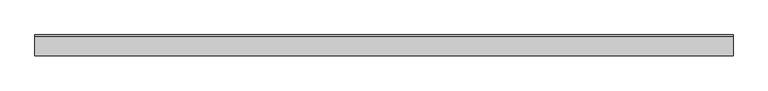
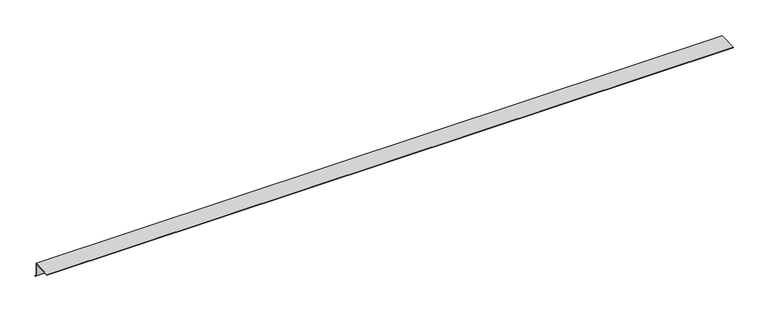
"""IFC4 building model written with IfcOpenShell, lengths in millimetres: proxy geometry, Generic Models 7:Generic Models 1:337419:Generic Models 1:337419 : Generic Models 7:Generic Models 1:337419:24 : Generic Models 7:Generic Models 1:337419:Generic Models 1:337419 : Generic Models 7:Generic Models 1:337419:301336."""

from ifc_helpers import new_model, si_unit, frame, origin, place, context, project, spatial, polyline, outline, extrude, source, transform, mapped, element, save


def generic_models_96069dc9(model_context):
    return source(origin(), model_context, "Body", "SweptSolid", [
        extrude(outline(polyline([(-536591.4802062, 10176.5740713), (-536591.5958611, 10179.3497879), (-536459.9713089, 10184.8341442), (-536459.9713089, 10095.8159785), (-536446.5009248, 10082.3455943), (-536448.4653558, 10080.3811633), (-536462.7494339, 10094.6652414), (-536462.7494339, 10181.9378535), (-536591.4802062, 10176.5740713)])), frame((591306.0367242, 0.0, 0.0), z_axis=(1.0, 0.0, 0.0), x_axis=(0.0, 1.0, 0.0)), (0.0, 0.0, 1.0), 4876.8),
    ])


if __name__ == "__main__":
    model = new_model("IFC4")
    model_context = context("Model", 3, world=origin())
    ifc_project = project(units=[si_unit("LENGTHUNIT", "METRE", prefix="MILLI")], contexts=[model_context])
    site = spatial("IfcSite", under=ifc_project)
    building = spatial("IfcBuilding", under=site)
    placement = place(None, origin())
    generic_models_shape = generic_models_96069dc9(model_context)
    element("IfcBuildingElementProxy", 1, Name="Generic Models 7:Generic Models 1:337419:Generic Models 1:337419 : Generic Models 7:Generic Models 1:337419:24 : Generic Models 7:Generic Models 1:337419:Generic Models 1:337419 : Generic Models 7:Generic Models 1:337419:301336", ObjectType="Generic Models 7:Generic Models 1:337419:Generic Models 1:337419 : Generic Models 7:Generic Models 1:337419:24 : Generic Models 7:Generic Models 1:337419:Generic Models 1:337419 : Generic Models 7:Generic Models 1:337419:301336", at=placement, inside=building, context=model_context, shape_type="MappedRepresentation", body=[
        mapped(generic_models_shape, transform((0.0, 0.0, 0.0), x_axis=(1.0, 0.0, 0.0), y_axis=(0.0, 1.0, 0.0), z_axis=(0.0, 0.0, 1.0))),
    ])
    save(model, "model.ifc")

# Revit data of these elements
# Type "Generic Models 7:Generic Models 1:337419:Generic Models 1:337419 : Generic Models 7:Generic Models 1:337419:24 : Generic Models 7:Generic Models 1:337419:Generic Models 1:337419 : Generic Models 7:Generic Models 1:337419:301336"
#   NameOverride = "Generic Models 7:Generic Models 1:337419:Generic Models 1:337419 : Generic Models 7:Generic Models 1:337419:301336"
#   ObjectTypeOverride = "Generic Models 1:337419 : Generic Models 7:Generic Models 1:337419"
#   Reference = "Generic Models 1"
#   Tag = "301336"
# Element 1 (IfcBuildingElementProxy, "Generic Models 7:Generic Models 1:337419:Generic Models 1:337419 : Generic Models 7:Generic Models 1:337419:24 : Generic Models 7:Generic Models 1:337419:Generic Models 1:337419 : Generic Models 7:Generic Models 1:337419:301336")
#   Materials on its faces: "BOX HIGH SIDE EAVE TRIM (FL-33)"
# Materials
#   "BOX HIGH SIDE EAVE TRIM (FL-33)": class "Generic", colour RGB 120 120 120, transparency 0, Cost = 0
